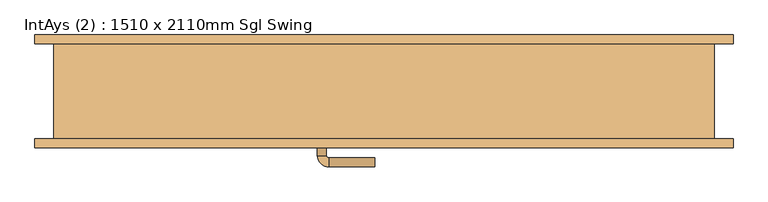
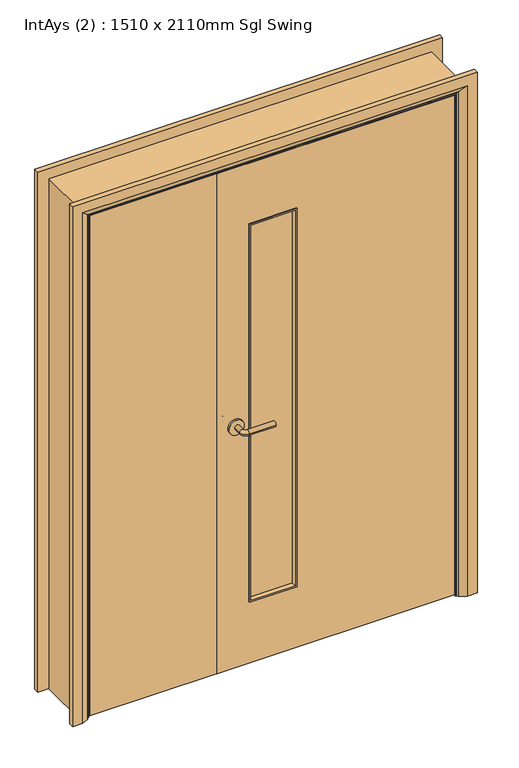
"""IFC4 building model written with IfcOpenShell, lengths in millimetres: door geometry, IntAys (2) : 1510 x 2110mm Sgl Swing."""

from ifc_helpers import new_model, si_unit, point, frame, frame_2d, origin, place, context, project, spatial, polyline, circle_curve, ellipse_curve, trimmed, segment, composite_curve, outline, extrude, faceted_brep, source, transform, mapped, element, save
from ifc_brep_helpers import plane_surface, cylinder_surface, revolved_surface, advanced_brep


def intays_2_1510_x_2110mm_sgl_swing_dce9c54a(model_context):
    return source(origin(), model_context, "Body", "SolidModel", [
        advanced_brep(
        [(88.5, -67.5, 1000.0), (108.5, -67.5, 1000.0), (88.5, -37.5, 1000.0), (108.5, -37.5, 1000.0), (113.5, -32.5, 1000.0), (113.5, -12.5, 1000.0), (218.5, -12.5, 1000.0), (218.5, -32.5, 1000.0)],
        [
            (0, 1, circle_curve(frame((98.5, -67.5, 1000.0), z_axis=(0.0, -1.0, 0.0), x_axis=(1.0, 0.0, 0.0)), 10.0)),
            (1, 0, circle_curve(frame((98.5, -67.5, 1000.0), z_axis=(0.0, -1.0, 0.0), x_axis=(1.0, 0.0, 0.0)), 10.0)),
            (0, 2),
            (2, 3, circle_curve(frame((98.5, -37.5, 1000.0), z_axis=(0.0, -1.0, 0.0), x_axis=(1.0, 0.0, 0.0)), 10.0)),
            (3, 1),
            (3, 2, circle_curve(frame((98.5, -37.5, 1000.0), z_axis=(0.0, -1.0, 0.0), x_axis=(1.0, 0.0, 0.0)), 10.0)),
            (4, 3, circle_curve(frame((113.5, -37.5, 1000.0), z_axis=(0.0, 0.0, 1.0), x_axis=(-1.0, 0.0, 0.0)), 5.0)),
            (2, 5, circle_curve(frame((113.5, -37.5, 1000.0), z_axis=(0.0, 0.0, -1.0), x_axis=(-1.0, 0.0, 0.0)), 25.0)),
            (5, 4, circle_curve(frame((113.5, -22.5, 1000.0), z_axis=(-1.0, 0.0, 0.0), x_axis=(0.0, -1.0, 0.0)), 10.0)),
            (4, 5, circle_curve(frame((113.5, -22.5, 1000.0), z_axis=(-1.0, 0.0, 0.0), x_axis=(0.0, -1.0, 0.0)), 10.0)),
            (6, 7, circle_curve(frame((218.5, -22.5, 1000.0), z_axis=(1.0, 0.0, 0.0), x_axis=(0.0, -1.0, 0.0)), 10.0)),
            (7, 6, circle_curve(frame((218.5, -22.5, 1000.0), z_axis=(1.0, 0.0, 0.0), x_axis=(0.0, -1.0, 0.0)), 10.0)),
            (5, 6),
            (7, 4),
        ],
        [
            plane_surface(frame((98.5, -67.5, 1000.0), z_axis=(0.0, -1.0, 0.0), x_axis=(0.0, 0.0, 1.0))),
            cylinder_surface(frame((98.5, -67.5, 1000.0), z_axis=(0.0, -1.0, 0.0), x_axis=(1.0, 0.0, 0.0)), 10.0),
            revolved_surface(trimmed(ellipse_curve(frame((98.5, -37.5, 1000.0), z_axis=(0.0, -1.0, 0.0), x_axis=(1.0, 0.0, 0.0)), 10.0, 10.0), [point((88.5, -37.5, 1000.0))], [point((108.5, -37.5, 1000.0))], True, "CARTESIAN"), (113.5, -37.5, 1000.0), (0.0, 0.0, -1.0)),
            revolved_surface(trimmed(ellipse_curve(frame((98.5, -37.5, 1000.0), z_axis=(0.0, -1.0, 0.0), x_axis=(1.0, 0.0, 0.0)), 10.0, 10.0), [point((108.5, -37.5, 1000.0))], [point((88.5, -37.5, 1000.0))], True, "CARTESIAN"), (113.5, -37.5, 1000.0), (0.0, 0.0, -1.0)),
            plane_surface(frame((218.5, -22.5, 1000.0), z_axis=(1.0, 0.0, 0.0), x_axis=(0.0, 0.0, 1.0))),
            cylinder_surface(frame((113.5, -22.5, 1000.0), z_axis=(-1.0, 0.0, 0.0), x_axis=(0.0, -1.0, 0.0)), 10.0),
        ],
        [
            (0, [[1, 2]]),
            (1, [[-1, 3, 4, 5]]),
            (1, [[-2, -5, 6, -3]]),
            (2, [[7, -4, 8, 9]]),
            (3, [[-8, -6, -7, 10]]),
            (4, [[11, 12]]),
            (5, [[-9, 13, -12, 14]]),
            (5, [[-10, -14, -11, -13]]),
        ],
    ),
        extrude(outline(composite_curve([segment(trimmed(circle_curve(frame_2d((1000.0, 96.0)), 30.0), [point((1000.0, 66.0))], [point((1000.0, 126.0))], False, "CARTESIAN"), True, "CONTINUOUS"), segment(trimmed(circle_curve(frame_2d((1000.0, 96.0)), 30.0), [point((1000.0, 126.0))], [point((1000.0, 66.0))], False, "CARTESIAN"), True, "CONTINUOUS")], self_intersect=False)), frame((0.0, -75.5, 0.0), z_axis=(0.0, 1.0, 0.0), x_axis=(0.0, 0.0, 1.0)), (0.0, 0.0, 1.0), 8.0),
        advanced_brep(
        [(88.5, -115.5, 1000.0), (108.5, -115.5, 1000.0), (108.5, -145.5, 1000.0), (88.5, -145.5, 1000.0), (113.5, -150.5, 1000.0), (113.5, -170.5, 1000.0), (218.5, -170.5, 1000.0), (218.5, -150.5, 1000.0)],
        [
            (0, 1, circle_curve(frame((98.5, -115.5, 1000.0), z_axis=(0.0, 1.0, 0.0), x_axis=(1.0, 0.0, 0.0)), 10.0)),
            (1, 0, circle_curve(frame((98.5, -115.5, 1000.0), z_axis=(0.0, 1.0, 0.0), x_axis=(1.0, 0.0, 0.0)), 10.0)),
            (1, 2),
            (2, 3, circle_curve(frame((98.5, -145.5, 1000.0), z_axis=(0.0, 1.0, 0.0), x_axis=(1.0, 0.0, 0.0)), 10.0)),
            (3, 0),
            (3, 2, circle_curve(frame((98.5, -145.5, 1000.0), z_axis=(0.0, 1.0, 0.0), x_axis=(1.0, 0.0, 0.0)), 10.0)),
            (4, 5, circle_curve(frame((113.5, -160.5, 1000.0), z_axis=(-1.0, 0.0, 0.0), x_axis=(0.0, 1.0, 0.0)), 10.0)),
            (5, 3, circle_curve(frame((113.5, -145.5, 1000.0), z_axis=(0.0, 0.0, -1.0), x_axis=(-1.0, 0.0, 0.0)), 25.0)),
            (2, 4, circle_curve(frame((113.5, -145.5, 1000.0), z_axis=(0.0, 0.0, 1.0), x_axis=(-1.0, 0.0, 0.0)), 5.0)),
            (5, 4, circle_curve(frame((113.5, -160.5, 1000.0), z_axis=(-1.0, 0.0, 0.0), x_axis=(0.0, 1.0, 0.0)), 10.0)),
            (6, 7, circle_curve(frame((218.5, -160.5, 1000.0), z_axis=(1.0, 0.0, 0.0), x_axis=(0.0, 1.0, 0.0)), 10.0)),
            (7, 6, circle_curve(frame((218.5, -160.5, 1000.0), z_axis=(1.0, 0.0, 0.0), x_axis=(0.0, 1.0, 0.0)), 10.0)),
            (4, 7),
            (6, 5),
        ],
        [
            plane_surface(frame((98.5, -115.5, 1000.0), z_axis=(0.0, 1.0, 0.0), x_axis=(0.0, 0.0, 1.0))),
            cylinder_surface(frame((98.5, -115.5, 1000.0), z_axis=(0.0, 1.0, 0.0), x_axis=(1.0, 0.0, 0.0)), 10.0),
            revolved_surface(trimmed(ellipse_curve(frame((98.5, -145.5, 1000.0), z_axis=(0.0, -1.0, 0.0), x_axis=(1.0, 0.0, 0.0)), 10.0, 10.0), [point((88.5, -145.5, 1000.0))], [point((108.5, -145.5, 1000.0))], True, "CARTESIAN"), (113.5, -145.5, 1000.0), (0.0, 0.0, -1.0)),
            revolved_surface(trimmed(ellipse_curve(frame((98.5, -145.5, 1000.0), z_axis=(0.0, -1.0, 0.0), x_axis=(1.0, 0.0, 0.0)), 10.0, 10.0), [point((108.5, -145.5, 1000.0))], [point((88.5, -145.5, 1000.0))], True, "CARTESIAN"), (113.5, -145.5, 1000.0), (0.0, 0.0, -1.0)),
            plane_surface(frame((218.5, -160.5, 1000.0), z_axis=(1.0, 0.0, 0.0), x_axis=(0.0, 0.0, 1.0))),
            cylinder_surface(frame((113.5, -160.5, 1000.0), z_axis=(-1.0, 0.0, 0.0), x_axis=(0.0, 1.0, 0.0)), 10.0),
        ],
        [
            (0, [[1, 2]]),
            (1, [[3, 4, 5, -2]]),
            (1, [[-5, 6, -3, -1]]),
            (2, [[7, 8, -4, 9]]),
            (3, [[10, -9, -6, -8]]),
            (4, [[11, 12]]),
            (5, [[13, -11, 14, -7]]),
            (5, [[-14, -12, -13, -10]]),
        ],
    ),
        extrude(outline(composite_curve([segment(trimmed(circle_curve(frame_2d((1000.0, 96.0)), 30.0), [point((1000.0, 66.0))], [point((1000.0, 126.0))], False, "CARTESIAN"), True, "CONTINUOUS"), segment(trimmed(circle_curve(frame_2d((1000.0, 96.0)), 30.0), [point((1000.0, 126.0))], [point((1000.0, 66.0))], False, "CARTESIAN"), True, "CONTINUOUS")], self_intersect=False)), frame((0.0, -115.5, 0.0), z_axis=(0.0, 1.0, 0.0), x_axis=(0.0, 0.0, 1.0)), (0.0, 0.0, 1.0), 8.0),
        extrude(outline(polyline([(2102.0, -508.0), (0.0, -508.0), (0.0, -476.0), (2070.0, -476.0), (2070.0, 954.0), (0.0, 954.0), (0.0, 986.0), (2102.0, 986.0), (2102.0, -508.0)])), frame((0.0, -107.5, 0.0), z_axis=(0.0, 1.0, 0.0), x_axis=(0.0, 0.0, 1.0)), (0.0, 0.0, 1.0), 215.0),
        advanced_brep(
        [(-551.0, 127.5, 0.0), (-511.0, 127.5, 0.0), (-485.0, 113.5, 0.0), (-481.0, 107.5, 0.0), (-551.0, 107.5, 0.0), (-551.0, 107.5, 2145.0), (-551.0, 127.5, 2145.0), (-481.0, 107.5, 2075.0), (959.0, 107.5, 2075.0), (959.0, 107.5, 0.0), (1029.0, 107.5, 0.0), (1029.0, 107.5, 2145.0), (-485.0, 113.5, 2079.0), (-511.0, 127.5, 2105.0), (1029.0, 127.5, 2145.0), (1029.0, 127.5, 0.0), (989.0, 127.5, 0.0), (989.0, 127.5, 2105.0), (963.0, 113.5, 0.0), (963.0, 113.5, 2079.0)],
        [
            (0, 1),
            (1, 2),
            (2, 3, circle_curve(frame((-489.0, 106.5, 0.0), z_axis=(0.0, 0.0, -1.0), x_axis=(-1.0, 0.0, 0.0)), 8.0622577)),
            (3, 4),
            (4, 0),
            (4, 5),
            (5, 6),
            (6, 0),
            (3, 7),
            (7, 8),
            (8, 9),
            (9, 10),
            (10, 11),
            (11, 5),
            (2, 12),
            (12, 7, ellipse_curve(frame((-489.0, 106.5, 2083.0), z_axis=(-0.7071067811865475, 0.0, -0.7071067811865475), x_axis=(0.7071067811865474, 0.0, -0.7071067811865476)), 11.4017543, 8.0622577)),
            (1, 13),
            (13, 12),
            (6, 14),
            (14, 15),
            (15, 16),
            (16, 17),
            (17, 13),
            (10, 15),
            (14, 11),
            (9, 18, circle_curve(frame((967.0, 106.5, 0.0), z_axis=(0.0, 0.0, -1.0), x_axis=(1.0, 0.0, 0.0)), 8.0622577)),
            (18, 16),
            (19, 18),
            (8, 19, ellipse_curve(frame((967.0, 106.5, 2083.0), z_axis=(0.7071067811865475, 0.0, -0.7071067811865475), x_axis=(0.7071067811865474, 0.0, 0.7071067811865476)), 11.4017543, 8.0622577)),
            (19, 17),
            (12, 19),
        ],
        [
            plane_surface(frame((-481.0, 107.5, 0.0), z_axis=(0.0, 0.0, -1.0), x_axis=(0.0, 1.0, 0.0))),
            plane_surface(frame((-551.0, 127.5, 0.0), z_axis=(-1.0, 0.0, 0.0), x_axis=(0.0, 0.0, 1.0))),
            plane_surface(frame((-551.0, 107.5, 0.0), z_axis=(0.0, -1.0, 0.0), x_axis=(0.0, 0.0, 1.0))),
            cylinder_surface(frame((-489.0, 106.5, 0.0), z_axis=(0.0, 0.0, -1.0), x_axis=(-1.0, 0.0, 0.0)), 8.0622577),
            plane_surface(frame((-485.0, 113.5, 0.0), z_axis=(0.4740998230350183, 0.8804710999221749, 0.0), x_axis=(0.0, 0.0, 1.0))),
            plane_surface(frame((-511.0, 127.5, 0.0), z_axis=(0.0, 1.0, 0.0), x_axis=(0.0, 0.0, 1.0))),
            plane_surface(frame((1029.0, 127.5, 2145.0), z_axis=(1.0, 0.0, 0.0), x_axis=(0.0, 0.0, -1.0))),
            plane_surface(frame((959.0, 107.5, 0.0), z_axis=(0.0, 0.0, -1.0), x_axis=(0.0, 1.0, 0.0))),
            cylinder_surface(frame((967.0, 106.5, 2075.0), z_axis=(0.0, 0.0, 1.0), x_axis=(1.0, 0.0, 0.0)), 8.0622577),
            plane_surface(frame((963.0, 113.5, 2079.0), z_axis=(-0.4740998230350183, 0.8804710999221749, 0.0), x_axis=(0.0, 0.0, -1.0))),
            plane_surface(frame((-551.0, 127.5, 2145.0), z_axis=(0.0, 0.0, 1.0), x_axis=(1.0, 0.0, 0.0))),
            cylinder_surface(frame((-481.0, 106.5, 2083.0), z_axis=(-1.0, 0.0, 0.0), x_axis=(0.0, 0.0, 1.0)), 8.0622577),
            plane_surface(frame((-485.0, 113.5, 2079.0), z_axis=(0.0, 0.8804710999221749, -0.4740998230350183), x_axis=(1.0, 0.0, 0.0))),
        ],
        [
            (0, [[1, 2, 3, 4, 5]]),
            (1, [[6, 7, 8, -5]]),
            (2, [[9, 10, 11, 12, 13, 14, -6, -4]]),
            (3, [[15, 16, -9, -3]]),
            (4, [[17, 18, -15, -2]]),
            (5, [[-8, 19, 20, 21, 22, 23, -17, -1]]),
            (6, [[-13, 24, -20, 25]]),
            (7, [[-24, -12, 26, 27, -21]]),
            (8, [[28, -26, -11, 29]]),
            (9, [[-22, -27, -28, 30]]),
            (10, [[-14, -25, -19, -7]]),
            (11, [[31, -29, -10, -16]]),
            (12, [[-23, -30, -31, -18]]),
        ],
    ),
        advanced_brep(
        [(1029.0, -127.5, 0.0), (989.0, -127.5, 0.0), (963.0, -113.5, 0.0), (959.0, -107.5, 0.0), (1029.0, -107.5, 0.0), (1029.0, -107.5, 2145.0), (1029.0, -127.5, 2145.0), (959.0, -107.5, 2075.0), (-481.0, -107.5, 2075.0), (-481.0, -107.5, 0.0), (-551.0, -107.5, 0.0), (-551.0, -107.5, 2145.0), (963.0, -113.5, 2079.0), (989.0, -127.5, 2105.0), (-551.0, -127.5, 2145.0), (-551.0, -127.5, 0.0), (-511.0, -127.5, 0.0), (-511.0, -127.5, 2105.0), (-485.0, -113.5, 0.0), (-485.0, -113.5, 2079.0)],
        [
            (0, 1),
            (1, 2),
            (2, 3, circle_curve(frame((967.0, -106.5, 0.0), z_axis=(0.0, 0.0, -1.0), x_axis=(1.0, 0.0, 0.0)), 8.0622577)),
            (3, 4),
            (4, 0),
            (4, 5),
            (5, 6),
            (6, 0),
            (3, 7),
            (7, 8),
            (8, 9),
            (9, 10),
            (10, 11),
            (11, 5),
            (2, 12),
            (12, 7, ellipse_curve(frame((967.0, -106.5, 2083.0), z_axis=(0.7071067811865475, 0.0, -0.7071067811865475), x_axis=(-0.7071067811865474, 0.0, -0.7071067811865476)), 11.4017543, 8.0622577)),
            (1, 13),
            (13, 12),
            (6, 14),
            (14, 15),
            (15, 16),
            (16, 17),
            (17, 13),
            (10, 15),
            (14, 11),
            (9, 18, circle_curve(frame((-489.0, -106.5, 0.0), z_axis=(0.0, 0.0, -1.0), x_axis=(-1.0, 0.0, 0.0)), 8.0622577)),
            (18, 16),
            (19, 18),
            (8, 19, ellipse_curve(frame((-489.0, -106.5, 2083.0), z_axis=(-0.7071067811865475, 0.0, -0.7071067811865475), x_axis=(-0.7071067811865474, 0.0, 0.7071067811865476)), 11.4017543, 8.0622577)),
            (19, 17),
            (12, 19),
        ],
        [
            plane_surface(frame((959.0, -107.5, 0.0), z_axis=(0.0, 0.0, -1.0), x_axis=(0.0, 1.0, 0.0))),
            plane_surface(frame((1029.0, -127.5, 0.0), z_axis=(1.0, 0.0, 0.0), x_axis=(0.0, 0.0, 1.0))),
            plane_surface(frame((1029.0, -107.5, 0.0), z_axis=(0.0, 1.0, 0.0), x_axis=(0.0, 0.0, 1.0))),
            cylinder_surface(frame((967.0, -106.5, 0.0), z_axis=(0.0, 0.0, -1.0), x_axis=(1.0, 0.0, 0.0)), 8.0622577),
            plane_surface(frame((963.0, -113.5, 0.0), z_axis=(-0.4740998230350126, -0.8804710999221779, 0.0), x_axis=(0.0, 0.0, 1.0))),
            plane_surface(frame((989.0, -127.5, 0.0), z_axis=(0.0, -1.0, 0.0), x_axis=(0.0, 0.0, 1.0))),
            plane_surface(frame((-551.0, -127.5, 2145.0), z_axis=(-1.0, 0.0, 0.0), x_axis=(0.0, 0.0, -1.0))),
            plane_surface(frame((-481.0, -107.5, 0.0), z_axis=(0.0, 0.0, -1.0), x_axis=(0.0, 1.0, 0.0))),
            cylinder_surface(frame((-489.0, -106.5, 2075.0), z_axis=(0.0, 0.0, 1.0), x_axis=(-1.0, 0.0, 0.0)), 8.0622577),
            plane_surface(frame((-485.0, -113.5, 2079.0), z_axis=(0.4740998230350183, -0.8804710999221749, 0.0), x_axis=(0.0, 0.0, -1.0))),
            plane_surface(frame((1029.0, -127.5, 2145.0), z_axis=(0.0, 0.0, 1.0), x_axis=(-1.0, 0.0, 0.0))),
            cylinder_surface(frame((959.0, -106.5, 2083.0), z_axis=(1.0, 0.0, 0.0), x_axis=(0.0, 0.0, 1.0)), 8.0622577),
            plane_surface(frame((963.0, -113.5, 2079.0), z_axis=(0.0, -0.8804710999221763, -0.4740998230350154), x_axis=(-1.0, 0.0, 0.0))),
        ],
        [
            (0, [[1, 2, 3, 4, 5]]),
            (1, [[6, 7, 8, -5]]),
            (2, [[9, 10, 11, 12, 13, 14, -6, -4]]),
            (3, [[15, 16, -9, -3]]),
            (4, [[17, 18, -15, -2]]),
            (5, [[-8, 19, 20, 21, 22, 23, -17, -1]]),
            (6, [[-13, 24, -20, 25]]),
            (7, [[-24, -12, 26, 27, -21]]),
            (8, [[28, -26, -11, 29]]),
            (9, [[-22, -27, -28, 30]]),
            (10, [[-14, -25, -19, -7]]),
            (11, [[31, -29, -10, -16]]),
            (12, [[-23, -30, -31, -18]]),
        ],
    ),
        faceted_brep([(-457.0, -72.5, 0.0), (-476.0, -72.5, 0.0), (-476.0, -40.5, 0.0), (-457.0, -40.5, 0.0), (-457.0, -40.5, 2051.0), (-457.0, -72.5, 2051.0), (-476.0, -40.5, 2070.0), (-476.0, -72.5, 2070.0), (935.0, -72.5, 0.0), (935.0, -40.5, 0.0), (954.0, -40.5, 0.0), (954.0, -72.5, 0.0), (935.0, -72.5, 2051.0), (954.0, -72.5, 2070.0), (954.0, -40.5, 2070.0), (935.0, -40.5, 2051.0)], [[[0, 1, 2, 3]], [[3, 4, 5, 0]], [[2, 6, 4, 3]], [[1, 7, 6, 2]], [[0, 5, 7, 1]], [[8, 9, 10, 11]], [[12, 8, 11, 13]], [[13, 11, 10, 14]], [[14, 10, 9, 15]], [[15, 9, 8, 12]], [[4, 15, 12, 5]], [[6, 14, 15, 4]], [[7, 13, 14, 6]], [[5, 12, 13, 7]]]),
        extrude(outline(polyline([(335.0, -85.5), (335.0, -97.5), (150.0, -97.5), (150.0, -85.5), (335.0, -85.5)])), frame((0.0, 0.0, 257.0), z_axis=(0.0, 0.0, 1.0), x_axis=(1.0, 0.0, 0.0)), (0.0, 0.0, 1.0), 1560.0),
        extrude(outline(polyline([(22.0, -75.5), (22.0, -107.5), (-473.0, -107.5), (-473.0, -75.5), (22.0, -75.5)])), frame((0.0, 0.0, 5.753223), z_axis=(0.0, 0.0, 1.0), x_axis=(1.0, 0.0, 0.0)), (0.0, 0.0, 1.0), 2061.246777),
        extrude(outline(polyline([(5.753223, 951.0), (2067.0, 951.0), (2067.0, 25.0), (5.753223, 25.0), (5.753223, 951.0)]), holes=[polyline([(1817.0, 150.0), (1817.0, 335.0), (257.0, 335.0), (257.0, 150.0), (1817.0, 150.0)])]), frame((0.0, -107.5, 0.0), z_axis=(0.0, 1.0, 0.0), x_axis=(0.0, 0.0, 1.0)), (0.0, 0.0, 1.0), 32.0),
        faceted_brep([(335.0, -72.5, 257.0), (335.0, -72.5, 1817.0), (335.0, -85.5, 1817.0), (335.0, -85.5, 257.0), (323.0, -85.5, 269.0), (323.0, -85.5, 1805.0), (329.0, -72.5, 1811.0), (329.0, -72.5, 263.0), (150.0, -72.5, 1817.0), (150.0, -85.5, 1817.0), (162.0, -85.5, 1805.0), (156.0, -72.5, 1811.0), (150.0, -72.5, 257.0), (150.0, -85.5, 257.0), (162.0, -85.5, 269.0), (156.0, -72.5, 263.0)], [[[0, 1, 2, 3]], [[4, 5, 6, 7]], [[1, 8, 9, 2]], [[5, 10, 11, 6]], [[8, 12, 13, 9]], [[10, 14, 15, 11]], [[3, 2, 9, 13], [5, 4, 14, 10]], [[12, 0, 3, 13]], [[1, 0, 12, 8], [7, 6, 11, 15]], [[14, 4, 7, 15]]]),
        faceted_brep([(150.0, -110.5, 257.0), (150.0, -110.5, 1817.0), (150.0, -97.5, 1817.0), (150.0, -97.5, 257.0), (162.0, -97.5, 269.0), (162.0, -97.5, 1805.0), (156.0, -110.5, 1811.0), (156.0, -110.5, 263.0), (335.0, -110.5, 1817.0), (335.0, -97.5, 1817.0), (323.0, -97.5, 1805.0), (329.0, -110.5, 1811.0), (335.0, -110.5, 257.0), (335.0, -97.5, 257.0), (323.0, -97.5, 269.0), (329.0, -110.5, 263.0)], [[[0, 1, 2, 3]], [[4, 5, 6, 7]], [[1, 8, 9, 2]], [[5, 10, 11, 6]], [[8, 12, 13, 9]], [[10, 14, 15, 11]], [[3, 2, 9, 13], [5, 4, 14, 10]], [[12, 0, 3, 13]], [[1, 0, 12, 8], [7, 6, 11, 15]], [[14, 4, 7, 15]]]),
    ])


if __name__ == "__main__":
    model = new_model("IFC4")
    model_context = context("Model", 3, world=origin())
    ifc_project = project(units=[si_unit("LENGTHUNIT", "METRE", prefix="MILLI")], contexts=[model_context])
    site = spatial("IfcSite", under=ifc_project)
    building = spatial("IfcBuilding", under=site)
    placement = place(None, origin())
    intays_2_1510_x_2110mm_sgl_swing_shape = intays_2_1510_x_2110mm_sgl_swing_dce9c54a(model_context)
    element("IfcDoor", 1, ObjectType="IntAys (2) : 1510 x 2110mm Sgl Swing", at=placement, inside=building, context=model_context, shape_type="MappedRepresentation", body=[
        mapped(intays_2_1510_x_2110mm_sgl_swing_shape, transform((0.0, 0.0, 0.0), x_axis=(1.0, 0.0, 0.0), y_axis=(0.0, 1.0, 0.0), z_axis=(0.0, 0.0, 1.0))),
    ])
    save(model, "model.ifc")

# Revit data of these elements
# Type "IntAys (2) : 1510 x 2110mm Sgl Swing"
#   Type Mark = "46"
#   Type Comments = "Internal Asymmetric"
#   Operation = "DoubleDoorSingleSwing"
#   Construction Type Id = "SGL"
#   Keynote = "L20"
#   Description = "Internal Asymmetric Door"
#   Analytic Construction = "Large single-glazed windows"
#   Visual Light Transmittance = 0.9
#   VisionPanel Width = 185 mm
#   Thickness = 32 mm
#   Stop Thickness = 19 mm
#   Stop Depth = 32 mm
#   Stile Top Rail = 250 mm
#   Stile Shutting = 125 mm
#   Stile Bottom Rail = 250 mm
#   Solar Heat Gain Coefficient = 0.86
#   Secondary Panel Width = 495 mm
#   Rough Width = 1510 mm
#   Rough Height = 2110 mm
#   Main Panel Width = 926 mm
#   Heat Transfer Coefficient (U) = 5.5617 W/(m²·K)
#   Handle Z Distance = 1000 mm
#   Handle X Distance = 75 mm
#   Handle Length = 350 mm
#   Frame Thickness = 32 mm
#   Door Panel Width = 926 mm
#   Door Panel Thickness = 32 mm
#   Height = 2110 mm
#   Door Panel Offset = 0 mm
#   Structural Tolerance = 8 mm
#   Tolerance = 3 mm
#   UnderCut = 7 mm
#   Width = 1510 mm
#   Door Panel Height = 2060 mm
#   Architrave Setback = 5 mm
#   Vis - Swing Single = yes
#   Vis - Swing Opposing = no
#   Vis - Swing Double = no
#   Vis - Stops = yes
#   Vis - Ironmongery = yes
#   Define Thermal Properties by = 1
#   Material Ironmongery = Door - Handle
#   Material Glass = Door - Glazing
#   Material Frame = Door - Frame/Mullion
#   Material Door = Door - Panel
#   Material Beading = Door - Panel
#   Material Architrave = Door - Architrave
#   Handle Style = element 261135
#   Function = (empty or 0)
#   Wall Closure = (empty or 0)
# Element 1 (IfcDoor, "IntAys (2) : 1510 x 2110mm Sgl Swing")
#   Materials on its faces: "Door - Panel", "Door - Architrave", "Door - Handle", "Door - Frame/Mullion", "Door - Glazing"
# Materials
#   "Door - Handle": class "Miscellaneous", colour RGB 0 0 0, transparency 0, Keynote = "P21"
#   "Door - Glazing": class "Miscellaneous", colour RGB 0 0 255, transparency 0.75
#   "Door - Frame/Mullion": class "Wood", colour RGB 212 179 113, transparency 0, Keynote = "L20"
#   "Door - Panel": class "Wood", colour RGB 210 159 95, transparency 0, Keynote = "L20"
#   "Door - Architrave": class "Wood", colour RGB 154 90 5, transparency 0, Keynote = "P20"
